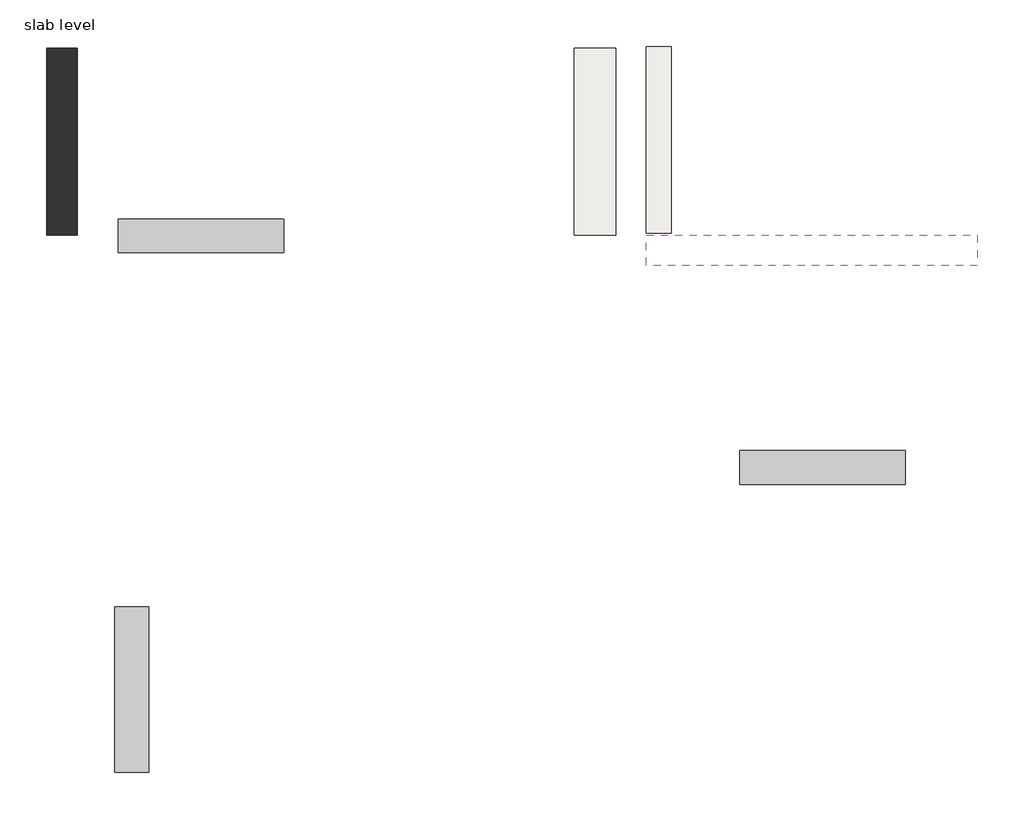
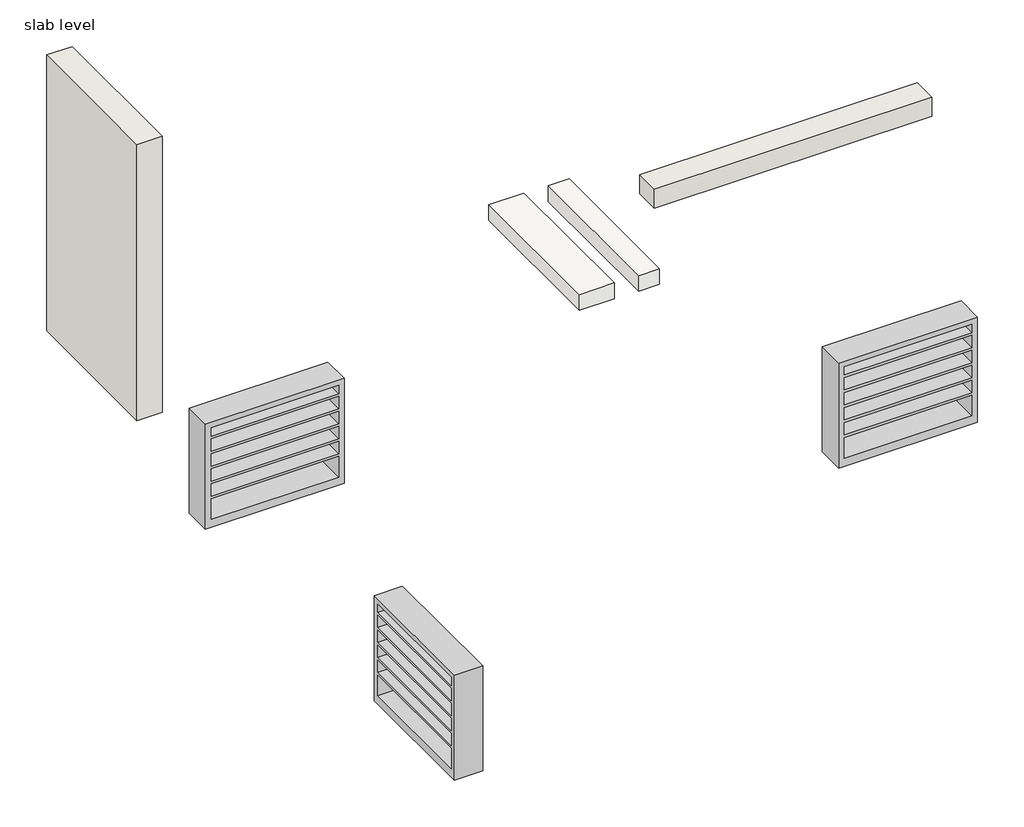
# One storey: 3 furniture elements, 2 slabs, 2 walls.
"""IFC4 building model written with IfcOpenShell, lengths in millimetres."""

import ifcopenshell
import ifcopenshell.guid

model = None  # the IFC model being written
_history = None  # IfcOwnerHistory: only IFC2X3 demands one
_inside = {}  # id of a spatial element -> (the spatial element, [elements in it])
_under = {}  # id of a project, library or spatial element -> (it, [spatial elements below it])
_declared = {}  # id of a project -> (the project, [libraries it declares])
_typed = {}  # id of a type object -> (the type object, [elements of that type])
_made_of = {}  # id of a material, layer set ... -> (it, [elements and type objects made of it])


def new_model(schema):
    """Start an empty IFC model of exactly this schema.

    Asked for "IFC4X3", IfcOpenShell would pick the latest addendum, in which some entities
    have other attributes; the version numbers below select the first issue.
    IFC2X3 requires an IfcOwnerHistory on every rooted entity: one is made here for all.
    """
    global model, _history
    if schema == "IFC4X3":
        model = ifcopenshell.file(schema_version=(4, 3, 0, 0))
    else:
        model = ifcopenshell.file(schema=schema)
    _inside.clear()
    _under.clear()
    _declared.clear()
    _typed.clear()
    _made_of.clear()
    _history = None
    if model.schema == "IFC2X3":
        org = make("IfcOrganization", Name="unknown")
        user = make(
            "IfcPersonAndOrganization",
            ThePerson=make("IfcPerson", FamilyName="unknown"),
            TheOrganization=org,
        )
        app = make(
            "IfcApplication",
            ApplicationDeveloper=org,
            Version="unknown",
            ApplicationFullName="unknown",
            ApplicationIdentifier="unknown",
        )
        _history = make(
            "IfcOwnerHistory",
            OwningUser=user,
            OwningApplication=app,
            ChangeAction="ADDED",
            CreationDate=0,
        )
    return model


def make(cls, **values):
    """One entity of the class cls with the attributes given. An attribute that is None is left unset."""
    return model.create_entity(
        cls, **{name: value for name, value in values.items() if value is not None}
    )


def rooted(cls, **values):
    """An entity with a GlobalId (a new one), such as an element, a storey or a relation."""
    return make(cls, GlobalId=ifcopenshell.guid.new(), OwnerHistory=_history, **values)


def si_unit(unit_type, name, prefix=None):
    """IfcSIUnit, for example si_unit("LENGTHUNIT", "METRE", prefix="MILLI")."""
    return make("IfcSIUnit", UnitType=unit_type, Prefix=prefix, Name=name)


def assignment(units):
    """IfcUnitAssignment: the units of a project."""
    return None if units is None else make("IfcUnitAssignment", Units=units)


def point(xyz):
    """IfcCartesianPoint."""
    return None if xyz is None else make("IfcCartesianPoint", Coordinates=xyz)


def direction(xyz):
    """IfcDirection."""
    return None if xyz is None else make("IfcDirection", DirectionRatios=xyz)


def frame(location, z_axis=None, x_axis=None):
    """IfcAxis2Placement3D, a coordinate frame: its origin and axes. An axis left out is left unset."""
    return make(
        "IfcAxis2Placement3D",
        Location=point(location),
        Axis=direction(z_axis),
        RefDirection=direction(x_axis),
    )


def origin():
    """The frame at (0, 0, 0) with its axes left unset."""
    return frame((0.0, 0.0, 0.0))


def place(relative_to, where):
    """IfcLocalPlacement: puts the frame where relative to a parent placement (None: the world)."""
    return make(
        "IfcLocalPlacement", PlacementRelTo=relative_to, RelativePlacement=where
    )


def context(
    kind, dimensions, precision=None, world=None, true_north=None, identifier=None
):
    """IfcGeometricRepresentationContext, for example the 3D "Model" context."""
    return make(
        "IfcGeometricRepresentationContext",
        ContextIdentifier=identifier,
        ContextType=kind,
        CoordinateSpaceDimension=dimensions,
        Precision=precision,
        WorldCoordinateSystem=world,
        TrueNorth=true_north,
    )


def project(units=None, contexts=None):
    """IfcProject with its units and contexts."""
    return rooted(
        "IfcProject",
        Name="project",
        RepresentationContexts=contexts,
        UnitsInContext=assignment(units),
    )


def spatial(cls, under=None, at=None, **own):
    """A site, building, storey or space (cls), placed at a placement, below another one or the project."""
    s = rooted(cls, ObjectPlacement=at, **own)
    if under is not None:
        _under.setdefault(under.id(), (under, []))[1].append(s)
    return s


def polyline(points):
    """IfcPolyline through the points."""
    return make("IfcPolyline", Points=[point(p) for p in points])


def outline(outer, holes=None, kind="AREA"):
    """IfcArbitraryClosedProfileDef: a profile drawn as a closed curve; with holes, ...WithVoids."""
    if holes is None:
        return make("IfcArbitraryClosedProfileDef", ProfileType=kind, OuterCurve=outer)
    return make(
        "IfcArbitraryProfileDefWithVoids",
        ProfileType=kind,
        OuterCurve=outer,
        InnerCurves=holes,
    )


def extrude(swept, where, along, depth):
    """IfcExtrudedAreaSolid: the profile swept, set in the frame where, extruded along a direction by depth."""
    return make(
        "IfcExtrudedAreaSolid",
        SweptArea=swept,
        Position=where,
        ExtrudedDirection=direction(along),
        Depth=depth,
    )


def faces_of(points, faces, orient=None, outer=None):
    """IfcFace entities. A face is a list of loops; a loop is a list of indices into points, from 0.

    orient and outer hold one flag for each loop. By default every Orientation is true, the
    first loop of a face is its IfcFaceOuterBound and the others are IfcFaceBound.
    """
    made = []
    for i, loops in enumerate(faces):
        bounds = []
        for j, loop in enumerate(loops):
            is_outer = j == 0 if outer is None else outer[i][j]
            bounds.append(
                make(
                    "IfcFaceOuterBound" if is_outer else "IfcFaceBound",
                    Bound=make("IfcPolyLoop", Polygon=[points[k] for k in loop]),
                    Orientation=True if orient is None else orient[i][j],
                )
            )
        made.append(make("IfcFace", Bounds=bounds))
    return made


def faceted_brep(points, faces, orient=None, outer=None, voids=None):
    """IfcFacetedBrep: a solid bounded by flat faces; with voids (closed shells), ...WithVoids."""
    shared = [point(p) for p in points]
    hull = make("IfcClosedShell", CfsFaces=faces_of(shared, faces, orient, outer))
    if voids is None:
        return make("IfcFacetedBrep", Outer=hull)
    return make(
        "IfcFacetedBrepWithVoids",
        Outer=hull,
        Voids=[
            make(cls, CfsFaces=faces_of(shared, fs, o, b)) for cls, fs, o, b in voids
        ],
    )


def shape(context_of_items, identifier, shape_type, items):
    """IfcShapeRepresentation: the items that make up one representation, for example the "Body"."""
    return make(
        "IfcShapeRepresentation",
        ContextOfItems=context_of_items,
        RepresentationIdentifier=identifier,
        RepresentationType=shape_type,
        Items=items,
    )


def source(mapping_origin, context_of_items, identifier, shape_type, items):
    """IfcRepresentationMap: a shape defined once, which mapped items show again and again."""
    return make(
        "IfcRepresentationMap",
        MappingOrigin=mapping_origin,
        MappedRepresentation=shape(context_of_items, identifier, shape_type, items),
    )


def transform(
    local_origin,
    x_axis=None,
    y_axis=None,
    z_axis=None,
    scale=None,
    scale2=None,
    scale3=None,
    uniform=True,
):
    """IfcCartesianTransformationOperator3D, or its non-uniform kind. x_axis, y_axis, z_axis: its Axis1, 2, 3."""
    if uniform:
        return make(
            "IfcCartesianTransformationOperator3D",
            Axis1=direction(x_axis),
            Axis2=direction(y_axis),
            LocalOrigin=point(local_origin),
            Scale=scale,
            Axis3=direction(z_axis),
        )
    return make(
        "IfcCartesianTransformationOperator3DnonUniform",
        Axis1=direction(x_axis),
        Axis2=direction(y_axis),
        LocalOrigin=point(local_origin),
        Scale=scale,
        Axis3=direction(z_axis),
        Scale2=scale2,
        Scale3=scale3,
    )


def mapped(mapping_source, mapping_target):
    """IfcMappedItem: shows the shape of a source again, moved by a transform."""
    return make(
        "IfcMappedItem", MappingSource=mapping_source, MappingTarget=mapping_target
    )


def made_of(thing, what):
    """Note that an element or type object is made of a material, layer set ...; save() writes the relation."""
    if what is not None:
        _made_of.setdefault(what.id(), (what, []))[1].append(thing)
    return thing


def element(
    cls,
    number,
    at=None,
    inside=None,
    cuts=None,
    type_object=None,
    material=None,
    context=None,
    identifier="Body",
    shape_type=None,
    held_by="IfcProductDefinitionShape",
    body=None,
    shapes=None,
    **own,
):
    """One element of the class cls, such as IfcWall. Its Tag is "e" and its number.

    at: its placement. inside: the storey or other place that contains it. cuts: it is an
    opening in that element (IfcRelVoidsElement). A single representation is given by context,
    identifier, shape_type and body (its items); several are given by shapes. held_by: the class
    of the entity that holds the representations. save() writes the other relations.
    """
    e = rooted(cls, Tag="e%d" % number, ObjectPlacement=at, **own)
    if body is not None:
        shapes = [shape(context, identifier, shape_type, body)]
    if shapes is not None:
        e.Representation = make(held_by, Representations=shapes)
    if inside is not None:
        _inside.setdefault(inside.id(), (inside, []))[1].append(e)
    if cuts is not None:
        rooted(
            "IfcRelVoidsElement", RelatingBuildingElement=cuts, RelatedOpeningElement=e
        )
    if type_object is not None:
        _typed.setdefault(type_object.id(), (type_object, []))[1].append(e)
    return made_of(e, material)


def aggregate(whole, parts):
    """IfcRelAggregates: a whole, such as a stair, and the parts it consists of."""
    return rooted("IfcRelAggregates", RelatingObject=whole, RelatedObjects=parts)


def save(model, path):
    """Write the relations noted so far, then the file.

    IfcRelAggregates (storeys below a building ...), IfcRelContainedInSpatialStructure (elements
    in a storey), IfcRelDefinesByType, IfcRelAssociatesMaterial and IfcRelDeclares: one each for
    every whole, place, type object, material and project.
    """
    for whole, parts in _under.values():
        aggregate(whole, parts)
    for where, things in _inside.values():
        rooted(
            "IfcRelContainedInSpatialStructure",
            RelatedElements=things,
            RelatingStructure=where,
        )
    for kind, things in _typed.values():
        rooted("IfcRelDefinesByType", RelatedObjects=things, RelatingType=kind)
    for what, things in _made_of.values():
        rooted("IfcRelAssociatesMaterial", RelatedObjects=things, RelatingMaterial=what)
    for by, libraries in _declared.values():
        rooted("IfcRelDeclares", RelatingContext=by, RelatedDefinitions=libraries)
    model.write(path)


def m_shelving_0915_x_0254_x_1830mm_07cf747d(model_context):
    return source(origin(), model_context, "Body", "SweptSolid", [
        extrude(outline(polyline([(0.0, 625.0), (1000.0, 625.0), (1000.0, -625.0), (0.0, -625.0), (0.0, 625.0)]), holes=[polyline([(949.2, 574.2), (869.8428571, 574.2), (869.8428571, -574.2), (949.2, -574.2), (949.2, 574.2)]), polyline([(76.2, 574.2), (76.2, -574.2), (273.0142857, -574.2), (273.0142857, 574.2), (76.2, 574.2)]), polyline([(584.1285714, -574.2), (701.5857143, -574.2), (701.5857143, 574.2), (584.1285714, 574.2), (584.1285714, -574.2)]), polyline([(844.4428571, 574.2), (726.9857143, 574.2), (726.9857143, -574.2), (844.4428571, -574.2), (844.4428571, 574.2)]), polyline([(558.7285714, 574.2), (441.2714286, 574.2), (441.2714286, -574.2), (558.7285714, -574.2), (558.7285714, 574.2)]), polyline([(415.8714286, 574.2), (298.4142857, 574.2), (298.4142857, -574.2), (415.8714286, -574.2), (415.8714286, 574.2)])]), frame((0.0, -431.8, 0.0), z_axis=(0.0, 1.0, 0.0), x_axis=(0.0, 0.0, 1.0)), (0.0, 0.0, 1.0), 254.0),
    ])


model = new_model("IFC4")

# Units and contexts
model_context = context("Model", 3, world=origin())
ifc_project = project(units=[si_unit("LENGTHUNIT", "METRE", prefix="MILLI")], contexts=[model_context])

# Site, building, storey
site = spatial("IfcSite", under=ifc_project)
building = spatial("IfcBuilding", under=site)
storey = spatial("IfcBuildingStorey", under=building, Name="slab level", Elevation=1650.0)

# Furniture
placement = place(None, origin())
m_shelving_0915_x_0254_x_1830mm_shape = m_shelving_0915_x_0254_x_1830mm_07cf747d(model_context)
element("IfcFurniture", 1, ObjectType="M_Shelving : 0915 x 0254 x 1830mm", at=placement, inside=storey, context=model_context, shape_type="MappedRepresentation", body=[
    mapped(m_shelving_0915_x_0254_x_1830mm_shape, transform((5338.7310897, -5069.2919993, 1650.0), x_axis=(1.0, 0.0, 0.0), y_axis=(0.0, 1.0, 0.0), z_axis=(0.0, 0.0, 1.0))),
])
element("IfcFurniture", 2, ObjectType="M_Shelving : 0915 x 0254 x 1830mm", at=placement, inside=storey, context=model_context, shape_type="MappedRepresentation", body=[
    mapped(m_shelving_0915_x_0254_x_1830mm_shape, transform((425.6989616, -7053.1164349, 1650.0), x_axis=(0.0, -1.0000000000000002, 0.0), y_axis=(1.0000000000000002, 0.0, 0.0), z_axis=(0.0, 0.0, 1.0))),
])
element("IfcFurniture", 3, ObjectType="M_Shelving : 0915 x 0254 x 1830mm", at=placement, inside=storey, context=model_context, shape_type="MappedRepresentation", body=[
    mapped(m_shelving_0915_x_0254_x_1830mm_shape, transform((643.6629754, -3928.8919993, 1650.0), x_axis=(-1.0, 0.0, 0.0), y_axis=(0.0, -1.0, 0.0), z_axis=(0.0, 0.0, 1.0))),
])

# Slabs
element("IfcSlab", 4, ObjectType="Generic 150mm", at=placement, inside=storey, context=model_context, shape_type="SweptSolid", body=[
    extrude(outline(polyline([(4193.7449602, -2193.0129118), (4193.7449602, -3603.0129118), (4007.972444, -3603.0129118), (4007.972444, -2193.0129118), (4193.7449602, -2193.0129118)])), frame((0.0, 0.0, 2429.7891896), z_axis=(0.0, 0.0, 1.0), x_axis=(1.0, 0.0, 0.0)), (0.0, 0.0, 1.0), 150.0),
])
element("IfcSlab", 5, ObjectType="Generic 150mm", at=placement, inside=storey, context=model_context, shape_type="SweptSolid", body=[
    extrude(outline(polyline([(3777.8989616, -2207.0919993), (3777.8989616, -3617.0919993), (3464.2489616, -3617.0919993), (3464.2489616, -2207.0919993), (3777.8989616, -2207.0919993)])), frame((0.0, 0.0, 2448.0547198), z_axis=(0.0, 0.0, 1.0), x_axis=(1.0, 0.0, 0.0)), (0.0, 0.0, 1.0), 150.0),
])

# Walls
element("IfcWall", 6, ObjectType="wall 24", at=placement, inside=storey, context=model_context, shape_type="Brep", body=[
    faceted_brep([(-292.1010384, -3617.0919993, 5420.111043), (-292.1010384, -3617.0919993, 3550.0), (-292.1010384, -3617.0919993, 2792.7393231), (-292.1010384, -2207.0919993, 2792.7393231), (-292.1010384, -2207.0919993, 3550.0), (-292.1010384, -2207.0919993, 5420.111043), (-522.1010384, -3617.0919993, 2792.7393231), (-522.1010384, -3617.0919993, 5420.111043), (-522.1010384, -2207.0919993, 5420.111043), (-522.1010384, -2207.0919993, 2792.7393231)], [[[0, 1, 2, 3, 4, 5]], [[6, 7, 8, 9]], [[3, 2, 6, 9]], [[0, 5, 8, 7]], [[3, 9, 8, 5, 4]], [[0, 7, 6, 2, 1]]]),
])
element("IfcWall", 7, ObjectType="wall 24", at=placement, inside=storey, context=model_context, shape_type="SweptSolid", body=[
    extrude(outline(polyline([(6507.8989616, -3847.0919993), (4007.8989616, -3847.0919993), (4007.8989616, -3617.0919993), (6507.8989616, -3617.0919993), (6507.8989616, -3847.0919993)])), frame((0.0, 0.0, 3368.7323471), z_axis=(0.0, 0.0, 1.0), x_axis=(1.0, 0.0, 0.0)), (0.0, 0.0, 1.0), 181.2676529),
])

save(model, "model.ifc")

# Revit data of these elements
# Project information
#   Project Issue Date = "Issue Date"
#   Project Status = "Project Status"
#   Client Name = "Owner"
#   Project Address = "Enter address here"
#   Project Name = "Project Name"
#   Project Number = "0001"
# Type "M_Shelving : 0915 x 0254 x 1830mm"
#   Depth = 0.254 m
#   Height = 1 m
#   Width = 1.25 m
#   Material = Birch
# Type "Generic 150mm"
#   Function = 0
#   Layers, outside or top first: 0.15 m no material (function 1)
# Type "wall 24"
#   Layers, outside or top first: 0.01 m no material (function 1); 0.2 m no material (function 1); 0.02 m no material (function 1)
# Elements 1, 2, 3 (IfcFurniture, "M_Shelving : 0915 x 0254 x 1830mm")
#   Phase Created = New Construction
#   Materials on its faces: "Birch"
# Element 4 (IfcSlab, "Generic 150mm")
#   Comments = ""
#   Height Offset From Level = 0.929789 m
#   built-in parameter 1001954 = 1
#   Phase Created = New Construction
#   Materials on its faces: "Ceramic Tile", "Default Floor"
# Element 5 (IfcSlab, "Generic 150mm")
#   Comments = ""
#   Height Offset From Level = 0.948055 m
#   built-in parameter 1001954 = 1
#   Phase Created = New Construction
#   Materials on its faces: "Ceramic Tile", "Default Floor"
# Element 6 (IfcWall, "wall 24")
#   built-in parameter 1001111 = 1.142739 m
#   Top Offset = 0 m
#   Base Offset = 1.142739 m
#   Unconnected Height = 2.627372 m
#   wall height = 2.627372 m
#   Phase Created = New Construction
#   Base Constraint = slab level
#   Materials on its faces: "Default Wall"
# Element 7 (IfcWall, "wall 24")
#   built-in parameter 1001111 = 1.718732 m
#   Top Offset = 0 m
#   Base Offset = 1.718732 m
#   Unconnected Height = 0.181268 m
#   wall height = 0.181268 m
#   Phase Created = New Construction
#   Base Constraint = slab level
#   Materials on its faces: "Default Wall"
# Materials
#   "Birch": class "Wood", colour RGB 224 178 126, transparency 0, Description = "Betula Alleghaniensis", Cost = 0
#   "Ceramic Tile": class "Ceramic", colour RGB 246 230 196, transparency 0, Description = "physical material", Cost = 0
#   "Default Floor": class "Miscellaneous", colour RGB 127 127 127, transparency 0, Cost = 0
#   "Default Wall": class "Miscellaneous", colour RGB 128 128 128, transparency 0, Cost = 0
